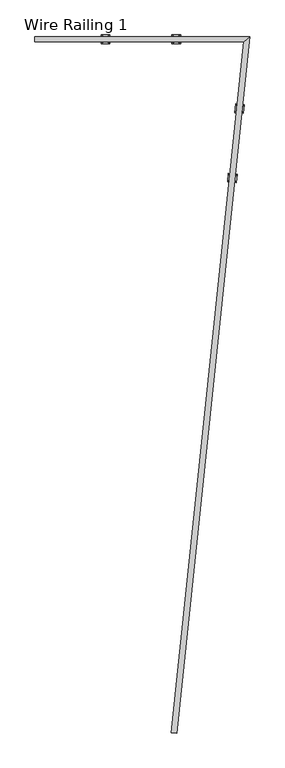
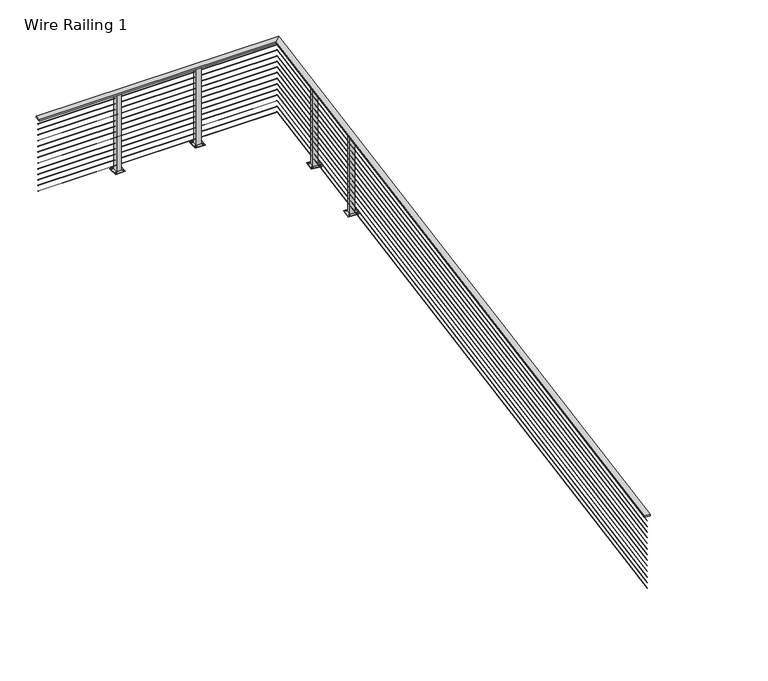
"""IFC4 building model written with IfcOpenShell, lengths in millimetres: railing geometry, Wire Railing 1."""

from ifc_helpers import new_model, si_unit, point, frame, frame_2d, origin, place, context, project, spatial, polyline, circle_curve, ellipse_curve, trimmed, segment, composite_curve, outline, extrude, faceted_brep, source, transform, mapped, element, save
from ifc_brep_helpers import plane_surface, cylinder_surface, advanced_brep


def wire_railing_1_cf5217c8(model_context):
    return source(origin(), model_context, "Body", "SolidModel", [
        faceted_brep([(32254.6127201, 40849.4411612, 270325.85), (32254.6127201, 40925.6411612, 270325.85), (32254.6127201, 40925.6411612, 270306.8), (32254.6127201, 40849.4411612, 270306.8), (35287.8207531, 40849.4411612, 270306.8), (35287.8207531, 40849.4411612, 270325.85), (35372.4494268, 40925.6411612, 270306.8), (35372.4494268, 40925.6411612, 270325.85), (34234.7001024, 30829.6674754, 270325.85), (34234.7001024, 30829.6674754, 270306.8), (34310.4826708, 30821.7024065, 270306.8), (34310.4826708, 30821.7024065, 270325.85)], [[[0, 1, 2, 3]], [[4, 5, 0, 3]], [[6, 4, 3, 2]], [[7, 6, 2, 1]], [[5, 7, 1, 0]], [[8, 9, 10, 11]], [[9, 8, 5, 4]], [[10, 9, 4, 6]], [[11, 10, 6, 7]], [[8, 11, 7, 5]]]),
        advanced_brep(
        [(32254.6127201, 40889.9224112, 270247.26875), (32254.6127201, 40885.1599112, 270247.26875), (35327.4904439, 40885.1599112, 270247.26875), (35332.779736, 40889.9224112, 270247.26875), (34274.9595918, 30825.4360325, 270247.26875), (34270.2231813, 30825.9338493, 270247.26875)],
        [
            (0, 1, circle_curve(frame((32254.6127201, 40887.5411612, 270247.26875), z_axis=(-1.0, 0.0, 0.0), x_axis=(0.0, -1.0, 0.0)), 2.38125)),
            (1, 0, circle_curve(frame((32254.6127201, 40887.5411612, 270247.26875), z_axis=(-1.0, 0.0, 0.0), x_axis=(0.0, -1.0, 0.0)), 2.38125)),
            (2, 3, ellipse_curve(frame((35330.13509, 40887.5411612, 270247.26875), z_axis=(-0.669130606358848, 0.7431448254774035, 0.0), x_axis=(0.7431448254774035, 0.6691306063588481, 0.0)), 3.5587223, 2.38125)),
            (3, 0),
            (1, 2),
            (3, 2, ellipse_curve(frame((35330.13509, 40887.5411612, 270247.26875), z_axis=(-0.669130606358848, 0.7431448254774035, 0.0), x_axis=(0.7431448254774035, 0.6691306063588481, 0.0)), 3.5587223, 2.38125)),
            (4, 5, circle_curve(frame((34272.5913866, 30825.6849409, 270247.26875), z_axis=(-0.10452846326767264, -0.9945218953682714, 0.0), x_axis=(-0.9945218953682714, 0.10452846326767264, 0.0)), 2.38125)),
            (5, 4, circle_curve(frame((34272.5913866, 30825.6849409, 270247.26875), z_axis=(-0.10452846326767264, -0.9945218953682714, 0.0), x_axis=(-0.9945218953682714, 0.10452846326767264, 0.0)), 2.38125)),
            (4, 3),
            (2, 5),
        ],
        [
            plane_surface(frame((32254.6127201, 40887.5411612, 270249.65), z_axis=(-1.0, 0.0, 0.0), x_axis=(0.0, -1.0, 0.0))),
            cylinder_surface(frame((35330.13509, 40887.5411612, 270247.26875), z_axis=(1.0, 0.0, 0.0), x_axis=(0.0, -1.0, 0.0)), 2.38125),
            plane_surface(frame((34272.5913866, 30825.6849409, 270249.65), z_axis=(-0.10452846326767265, -0.9945218953682714, 0.0), x_axis=(0.9945218953682714, -0.10452846326767265, 0.0))),
            cylinder_surface(frame((34272.5913866, 30825.6849409, 270247.26875), z_axis=(-0.10452846326767264, -0.9945218953682714, 0.0), x_axis=(-0.9945218953682714, 0.10452846326767264, 0.0)), 2.38125),
        ],
        [
            (0, [[1, 2]]),
            (1, [[3, 4, -2, 5]]),
            (1, [[6, -5, -1, -4]]),
            (2, [[7, 8]]),
            (3, [[-7, 9, -3, 10]]),
            (3, [[-8, -10, -6, -9]]),
        ],
    ),
        advanced_brep(
        [(32254.6127201, 40889.9224112, 270171.06875), (32254.6127201, 40885.1599112, 270171.06875), (35327.4904439, 40885.1599112, 270171.06875), (35332.779736, 40889.9224112, 270171.06875), (34274.9595918, 30825.4360325, 270171.06875), (34270.2231813, 30825.9338493, 270171.06875)],
        [
            (0, 1, circle_curve(frame((32254.6127201, 40887.5411612, 270171.06875), z_axis=(-1.0, 0.0, 0.0), x_axis=(0.0, -1.0, 0.0)), 2.38125)),
            (1, 0, circle_curve(frame((32254.6127201, 40887.5411612, 270171.06875), z_axis=(-1.0, 0.0, 0.0), x_axis=(0.0, -1.0, 0.0)), 2.38125)),
            (2, 3, ellipse_curve(frame((35330.13509, 40887.5411612, 270171.06875), z_axis=(-0.669130606358848, 0.7431448254774035, 0.0), x_axis=(0.7431448254774035, 0.6691306063588481, 0.0)), 3.5587223, 2.38125)),
            (3, 0),
            (1, 2),
            (3, 2, ellipse_curve(frame((35330.13509, 40887.5411612, 270171.06875), z_axis=(-0.669130606358848, 0.7431448254774035, 0.0), x_axis=(0.7431448254774035, 0.6691306063588481, 0.0)), 3.5587223, 2.38125)),
            (4, 5, circle_curve(frame((34272.5913866, 30825.6849409, 270171.06875), z_axis=(-0.10452846326767264, -0.9945218953682714, 0.0), x_axis=(-0.9945218953682714, 0.10452846326767264, 0.0)), 2.38125)),
            (5, 4, circle_curve(frame((34272.5913866, 30825.6849409, 270171.06875), z_axis=(-0.10452846326767264, -0.9945218953682714, 0.0), x_axis=(-0.9945218953682714, 0.10452846326767264, 0.0)), 2.38125)),
            (4, 3),
            (2, 5),
        ],
        [
            plane_surface(frame((32254.6127201, 40887.5411612, 270173.45), z_axis=(-1.0, 0.0, 0.0), x_axis=(0.0, -1.0, 0.0))),
            cylinder_surface(frame((35330.13509, 40887.5411612, 270171.06875), z_axis=(1.0, 0.0, 0.0), x_axis=(0.0, -1.0, 0.0)), 2.38125),
            plane_surface(frame((34272.5913866, 30825.6849409, 270173.45), z_axis=(-0.10452846326767265, -0.9945218953682714, 0.0), x_axis=(0.9945218953682714, -0.10452846326767265, 0.0))),
            cylinder_surface(frame((34272.5913866, 30825.6849409, 270171.06875), z_axis=(-0.10452846326767264, -0.9945218953682714, 0.0), x_axis=(-0.9945218953682714, 0.10452846326767264, 0.0)), 2.38125),
        ],
        [
            (0, [[1, 2]]),
            (1, [[3, 4, -2, 5]]),
            (1, [[6, -5, -1, -4]]),
            (2, [[7, 8]]),
            (3, [[-7, 9, -3, 10]]),
            (3, [[-8, -10, -6, -9]]),
        ],
    ),
        advanced_brep(
        [(32254.6127201, 40889.9224112, 270094.86875), (32254.6127201, 40885.1599112, 270094.86875), (35327.4904439, 40885.1599112, 270094.86875), (35332.779736, 40889.9224112, 270094.86875), (34274.9595918, 30825.4360325, 270094.86875), (34270.2231813, 30825.9338493, 270094.86875)],
        [
            (0, 1, circle_curve(frame((32254.6127201, 40887.5411612, 270094.86875), z_axis=(-1.0, 0.0, 0.0), x_axis=(0.0, -1.0, 0.0)), 2.38125)),
            (1, 0, circle_curve(frame((32254.6127201, 40887.5411612, 270094.86875), z_axis=(-1.0, 0.0, 0.0), x_axis=(0.0, -1.0, 0.0)), 2.38125)),
            (2, 3, ellipse_curve(frame((35330.13509, 40887.5411612, 270094.86875), z_axis=(-0.669130606358848, 0.7431448254774035, 0.0), x_axis=(0.7431448254774035, 0.6691306063588481, 0.0)), 3.5587223, 2.38125)),
            (3, 0),
            (1, 2),
            (3, 2, ellipse_curve(frame((35330.13509, 40887.5411612, 270094.86875), z_axis=(-0.669130606358848, 0.7431448254774035, 0.0), x_axis=(0.7431448254774035, 0.6691306063588481, 0.0)), 3.5587223, 2.38125)),
            (4, 5, circle_curve(frame((34272.5913866, 30825.6849409, 270094.86875), z_axis=(-0.10452846326767264, -0.9945218953682714, 0.0), x_axis=(-0.9945218953682714, 0.10452846326767264, 0.0)), 2.38125)),
            (5, 4, circle_curve(frame((34272.5913866, 30825.6849409, 270094.86875), z_axis=(-0.10452846326767264, -0.9945218953682714, 0.0), x_axis=(-0.9945218953682714, 0.10452846326767264, 0.0)), 2.38125)),
            (4, 3),
            (2, 5),
        ],
        [
            plane_surface(frame((32254.6127201, 40887.5411612, 270097.25), z_axis=(-1.0, 0.0, 0.0), x_axis=(0.0, -1.0, 0.0))),
            cylinder_surface(frame((35330.13509, 40887.5411612, 270094.86875), z_axis=(1.0, 0.0, 0.0), x_axis=(0.0, -1.0, 0.0)), 2.38125),
            plane_surface(frame((34272.5913866, 30825.6849409, 270097.25), z_axis=(-0.10452846326767265, -0.9945218953682714, 0.0), x_axis=(0.9945218953682714, -0.10452846326767265, 0.0))),
            cylinder_surface(frame((34272.5913866, 30825.6849409, 270094.86875), z_axis=(-0.10452846326767264, -0.9945218953682714, 0.0), x_axis=(-0.9945218953682714, 0.10452846326767264, 0.0)), 2.38125),
        ],
        [
            (0, [[1, 2]]),
            (1, [[3, 4, -2, 5]]),
            (1, [[6, -5, -1, -4]]),
            (2, [[7, 8]]),
            (3, [[-7, 9, -3, 10]]),
            (3, [[-8, -10, -6, -9]]),
        ],
    ),
        advanced_brep(
        [(32254.6127201, 40889.9224112, 270018.66875), (32254.6127201, 40885.1599112, 270018.66875), (35327.4904439, 40885.1599112, 270018.66875), (35332.779736, 40889.9224112, 270018.66875), (34274.9595918, 30825.4360325, 270018.66875), (34270.2231813, 30825.9338493, 270018.66875)],
        [
            (0, 1, circle_curve(frame((32254.6127201, 40887.5411612, 270018.66875), z_axis=(-1.0, 0.0, 0.0), x_axis=(0.0, -1.0, 0.0)), 2.38125)),
            (1, 0, circle_curve(frame((32254.6127201, 40887.5411612, 270018.66875), z_axis=(-1.0, 0.0, 0.0), x_axis=(0.0, -1.0, 0.0)), 2.38125)),
            (2, 3, ellipse_curve(frame((35330.13509, 40887.5411612, 270018.66875), z_axis=(-0.669130606358848, 0.7431448254774035, 0.0), x_axis=(0.7431448254774035, 0.6691306063588481, 0.0)), 3.5587223, 2.38125)),
            (3, 0),
            (1, 2),
            (3, 2, ellipse_curve(frame((35330.13509, 40887.5411612, 270018.66875), z_axis=(-0.669130606358848, 0.7431448254774035, 0.0), x_axis=(0.7431448254774035, 0.6691306063588481, 0.0)), 3.5587223, 2.38125)),
            (4, 5, circle_curve(frame((34272.5913866, 30825.6849409, 270018.66875), z_axis=(-0.10452846326767264, -0.9945218953682714, 0.0), x_axis=(-0.9945218953682714, 0.10452846326767264, 0.0)), 2.38125)),
            (5, 4, circle_curve(frame((34272.5913866, 30825.6849409, 270018.66875), z_axis=(-0.10452846326767264, -0.9945218953682714, 0.0), x_axis=(-0.9945218953682714, 0.10452846326767264, 0.0)), 2.38125)),
            (4, 3),
            (2, 5),
        ],
        [
            plane_surface(frame((32254.6127201, 40887.5411612, 270021.05), z_axis=(-1.0, 0.0, 0.0), x_axis=(0.0, -1.0, 0.0))),
            cylinder_surface(frame((35330.13509, 40887.5411612, 270018.66875), z_axis=(1.0, 0.0, 0.0), x_axis=(0.0, -1.0, 0.0)), 2.38125),
            plane_surface(frame((34272.5913866, 30825.6849409, 270021.05), z_axis=(-0.10452846326767265, -0.9945218953682714, 0.0), x_axis=(0.9945218953682714, -0.10452846326767265, 0.0))),
            cylinder_surface(frame((34272.5913866, 30825.6849409, 270018.66875), z_axis=(-0.10452846326767264, -0.9945218953682714, 0.0), x_axis=(-0.9945218953682714, 0.10452846326767264, 0.0)), 2.38125),
        ],
        [
            (0, [[1, 2]]),
            (1, [[3, 4, -2, 5]]),
            (1, [[6, -5, -1, -4]]),
            (2, [[7, 8]]),
            (3, [[-7, 9, -3, 10]]),
            (3, [[-8, -10, -6, -9]]),
        ],
    ),
        advanced_brep(
        [(32254.6127201, 40889.9224112, 269942.46875), (32254.6127201, 40885.1599112, 269942.46875), (35327.4904439, 40885.1599112, 269942.46875), (35332.779736, 40889.9224112, 269942.46875), (34274.9595918, 30825.4360325, 269942.46875), (34270.2231813, 30825.9338493, 269942.46875)],
        [
            (0, 1, circle_curve(frame((32254.6127201, 40887.5411612, 269942.46875), z_axis=(-1.0, 0.0, 0.0), x_axis=(0.0, -1.0, 0.0)), 2.38125)),
            (1, 0, circle_curve(frame((32254.6127201, 40887.5411612, 269942.46875), z_axis=(-1.0, 0.0, 0.0), x_axis=(0.0, -1.0, 0.0)), 2.38125)),
            (2, 3, ellipse_curve(frame((35330.13509, 40887.5411612, 269942.46875), z_axis=(-0.669130606358848, 0.7431448254774035, 0.0), x_axis=(0.7431448254774035, 0.6691306063588481, 0.0)), 3.5587223, 2.38125)),
            (3, 0),
            (1, 2),
            (3, 2, ellipse_curve(frame((35330.13509, 40887.5411612, 269942.46875), z_axis=(-0.669130606358848, 0.7431448254774035, 0.0), x_axis=(0.7431448254774035, 0.6691306063588481, 0.0)), 3.5587223, 2.38125)),
            (4, 5, circle_curve(frame((34272.5913866, 30825.6849409, 269942.46875), z_axis=(-0.10452846326767264, -0.9945218953682714, 0.0), x_axis=(-0.9945218953682714, 0.10452846326767264, 0.0)), 2.38125)),
            (5, 4, circle_curve(frame((34272.5913866, 30825.6849409, 269942.46875), z_axis=(-0.10452846326767264, -0.9945218953682714, 0.0), x_axis=(-0.9945218953682714, 0.10452846326767264, 0.0)), 2.38125)),
            (4, 3),
            (2, 5),
        ],
        [
            plane_surface(frame((32254.6127201, 40887.5411612, 269944.85), z_axis=(-1.0, 0.0, 0.0), x_axis=(0.0, -1.0, 0.0))),
            cylinder_surface(frame((35330.13509, 40887.5411612, 269942.46875), z_axis=(1.0, 0.0, 0.0), x_axis=(0.0, -1.0, 0.0)), 2.38125),
            plane_surface(frame((34272.5913866, 30825.6849409, 269944.85), z_axis=(-0.10452846326767265, -0.9945218953682714, 0.0), x_axis=(0.9945218953682714, -0.10452846326767265, 0.0))),
            cylinder_surface(frame((34272.5913866, 30825.6849409, 269942.46875), z_axis=(-0.10452846326767264, -0.9945218953682714, 0.0), x_axis=(-0.9945218953682714, 0.10452846326767264, 0.0)), 2.38125),
        ],
        [
            (0, [[1, 2]]),
            (1, [[3, 4, -2, 5]]),
            (1, [[6, -5, -1, -4]]),
            (2, [[7, 8]]),
            (3, [[-7, 9, -3, 10]]),
            (3, [[-8, -10, -6, -9]]),
        ],
    ),
        advanced_brep(
        [(32254.6127201, 40889.9224112, 269866.26875), (32254.6127201, 40885.1599112, 269866.26875), (35327.4904439, 40885.1599112, 269866.26875), (35332.779736, 40889.9224112, 269866.26875), (34274.9595918, 30825.4360325, 269866.26875), (34270.2231813, 30825.9338493, 269866.26875)],
        [
            (0, 1, circle_curve(frame((32254.6127201, 40887.5411612, 269866.26875), z_axis=(-1.0, 0.0, 0.0), x_axis=(0.0, -1.0, 0.0)), 2.38125)),
            (1, 0, circle_curve(frame((32254.6127201, 40887.5411612, 269866.26875), z_axis=(-1.0, 0.0, 0.0), x_axis=(0.0, -1.0, 0.0)), 2.38125)),
            (2, 3, ellipse_curve(frame((35330.13509, 40887.5411612, 269866.26875), z_axis=(-0.669130606358848, 0.7431448254774035, 0.0), x_axis=(0.7431448254774035, 0.6691306063588481, 0.0)), 3.5587223, 2.38125)),
            (3, 0),
            (1, 2),
            (3, 2, ellipse_curve(frame((35330.13509, 40887.5411612, 269866.26875), z_axis=(-0.669130606358848, 0.7431448254774035, 0.0), x_axis=(0.7431448254774035, 0.6691306063588481, 0.0)), 3.5587223, 2.38125)),
            (4, 5, circle_curve(frame((34272.5913866, 30825.6849409, 269866.26875), z_axis=(-0.10452846326767264, -0.9945218953682714, 0.0), x_axis=(-0.9945218953682714, 0.10452846326767264, 0.0)), 2.38125)),
            (5, 4, circle_curve(frame((34272.5913866, 30825.6849409, 269866.26875), z_axis=(-0.10452846326767264, -0.9945218953682714, 0.0), x_axis=(-0.9945218953682714, 0.10452846326767264, 0.0)), 2.38125)),
            (4, 3),
            (2, 5),
        ],
        [
            plane_surface(frame((32254.6127201, 40887.5411612, 269868.65), z_axis=(-1.0, 0.0, 0.0), x_axis=(0.0, -1.0, 0.0))),
            cylinder_surface(frame((35330.13509, 40887.5411612, 269866.26875), z_axis=(1.0, 0.0, 0.0), x_axis=(0.0, -1.0, 0.0)), 2.38125),
            plane_surface(frame((34272.5913866, 30825.6849409, 269868.65), z_axis=(-0.10452846326767265, -0.9945218953682714, 0.0), x_axis=(0.9945218953682714, -0.10452846326767265, 0.0))),
            cylinder_surface(frame((34272.5913866, 30825.6849409, 269866.26875), z_axis=(-0.10452846326767264, -0.9945218953682714, 0.0), x_axis=(-0.9945218953682714, 0.10452846326767264, 0.0)), 2.38125),
        ],
        [
            (0, [[1, 2]]),
            (1, [[3, 4, -2, 5]]),
            (1, [[6, -5, -1, -4]]),
            (2, [[7, 8]]),
            (3, [[-7, 9, -3, 10]]),
            (3, [[-8, -10, -6, -9]]),
        ],
    ),
        advanced_brep(
        [(32254.6127201, 40889.9224112, 269790.06875), (32254.6127201, 40885.1599112, 269790.06875), (35327.4904439, 40885.1599112, 269790.06875), (35332.779736, 40889.9224112, 269790.06875), (34274.9595918, 30825.4360325, 269790.06875), (34270.2231813, 30825.9338493, 269790.06875)],
        [
            (0, 1, circle_curve(frame((32254.6127201, 40887.5411612, 269790.06875), z_axis=(-1.0, 0.0, 0.0), x_axis=(0.0, -1.0, 0.0)), 2.38125)),
            (1, 0, circle_curve(frame((32254.6127201, 40887.5411612, 269790.06875), z_axis=(-1.0, 0.0, 0.0), x_axis=(0.0, -1.0, 0.0)), 2.38125)),
            (2, 3, ellipse_curve(frame((35330.13509, 40887.5411612, 269790.06875), z_axis=(-0.669130606358848, 0.7431448254774035, 0.0), x_axis=(0.7431448254774035, 0.6691306063588481, 0.0)), 3.5587223, 2.38125)),
            (3, 0),
            (1, 2),
            (3, 2, ellipse_curve(frame((35330.13509, 40887.5411612, 269790.06875), z_axis=(-0.669130606358848, 0.7431448254774035, 0.0), x_axis=(0.7431448254774035, 0.6691306063588481, 0.0)), 3.5587223, 2.38125)),
            (4, 5, circle_curve(frame((34272.5913866, 30825.6849409, 269790.06875), z_axis=(-0.10452846326767264, -0.9945218953682714, 0.0), x_axis=(-0.9945218953682714, 0.10452846326767264, 0.0)), 2.38125)),
            (5, 4, circle_curve(frame((34272.5913866, 30825.6849409, 269790.06875), z_axis=(-0.10452846326767264, -0.9945218953682714, 0.0), x_axis=(-0.9945218953682714, 0.10452846326767264, 0.0)), 2.38125)),
            (4, 3),
            (2, 5),
        ],
        [
            plane_surface(frame((32254.6127201, 40887.5411612, 269792.45), z_axis=(-1.0, 0.0, 0.0), x_axis=(0.0, -1.0, 0.0))),
            cylinder_surface(frame((35330.13509, 40887.5411612, 269790.06875), z_axis=(1.0, 0.0, 0.0), x_axis=(0.0, -1.0, 0.0)), 2.38125),
            plane_surface(frame((34272.5913866, 30825.6849409, 269792.45), z_axis=(-0.10452846326767265, -0.9945218953682714, 0.0), x_axis=(0.9945218953682714, -0.10452846326767265, 0.0))),
            cylinder_surface(frame((34272.5913866, 30825.6849409, 269790.06875), z_axis=(-0.10452846326767264, -0.9945218953682714, 0.0), x_axis=(-0.9945218953682714, 0.10452846326767264, 0.0)), 2.38125),
        ],
        [
            (0, [[1, 2]]),
            (1, [[3, 4, -2, 5]]),
            (1, [[6, -5, -1, -4]]),
            (2, [[7, 8]]),
            (3, [[-7, 9, -3, 10]]),
            (3, [[-8, -10, -6, -9]]),
        ],
    ),
        advanced_brep(
        [(32254.6127201, 40889.9224112, 269713.86875), (32254.6127201, 40885.1599112, 269713.86875), (35327.4904439, 40885.1599112, 269713.86875), (35332.779736, 40889.9224112, 269713.86875), (34274.9595918, 30825.4360325, 269713.86875), (34270.2231813, 30825.9338493, 269713.86875)],
        [
            (0, 1, circle_curve(frame((32254.6127201, 40887.5411612, 269713.86875), z_axis=(-1.0, 0.0, 0.0), x_axis=(0.0, -1.0, 0.0)), 2.38125)),
            (1, 0, circle_curve(frame((32254.6127201, 40887.5411612, 269713.86875), z_axis=(-1.0, 0.0, 0.0), x_axis=(0.0, -1.0, 0.0)), 2.38125)),
            (2, 3, ellipse_curve(frame((35330.13509, 40887.5411612, 269713.86875), z_axis=(-0.669130606358848, 0.7431448254774035, 0.0), x_axis=(0.7431448254774035, 0.6691306063588481, 0.0)), 3.5587223, 2.38125)),
            (3, 0),
            (1, 2),
            (3, 2, ellipse_curve(frame((35330.13509, 40887.5411612, 269713.86875), z_axis=(-0.669130606358848, 0.7431448254774035, 0.0), x_axis=(0.7431448254774035, 0.6691306063588481, 0.0)), 3.5587223, 2.38125)),
            (4, 5, circle_curve(frame((34272.5913866, 30825.6849409, 269713.86875), z_axis=(-0.10452846326767264, -0.9945218953682714, 0.0), x_axis=(-0.9945218953682714, 0.10452846326767264, 0.0)), 2.38125)),
            (5, 4, circle_curve(frame((34272.5913866, 30825.6849409, 269713.86875), z_axis=(-0.10452846326767264, -0.9945218953682714, 0.0), x_axis=(-0.9945218953682714, 0.10452846326767264, 0.0)), 2.38125)),
            (4, 3),
            (2, 5),
        ],
        [
            plane_surface(frame((32254.6127201, 40887.5411612, 269716.25), z_axis=(-1.0, 0.0, 0.0), x_axis=(0.0, -1.0, 0.0))),
            cylinder_surface(frame((35330.13509, 40887.5411612, 269713.86875), z_axis=(1.0, 0.0, 0.0), x_axis=(0.0, -1.0, 0.0)), 2.38125),
            plane_surface(frame((34272.5913866, 30825.6849409, 269716.25), z_axis=(-0.10452846326767265, -0.9945218953682714, 0.0), x_axis=(0.9945218953682714, -0.10452846326767265, 0.0))),
            cylinder_surface(frame((34272.5913866, 30825.6849409, 269713.86875), z_axis=(-0.10452846326767264, -0.9945218953682714, 0.0), x_axis=(-0.9945218953682714, 0.10452846326767264, 0.0)), 2.38125),
        ],
        [
            (0, [[1, 2]]),
            (1, [[3, 4, -2, 5]]),
            (1, [[6, -5, -1, -4]]),
            (2, [[7, 8]]),
            (3, [[-7, 9, -3, 10]]),
            (3, [[-8, -10, -6, -9]]),
        ],
    ),
        advanced_brep(
        [(32254.6127201, 40889.9224112, 269637.66875), (32254.6127201, 40885.1599112, 269637.66875), (35327.4904439, 40885.1599112, 269637.66875), (35332.779736, 40889.9224112, 269637.66875), (34274.9595918, 30825.4360325, 269637.66875), (34270.2231813, 30825.9338493, 269637.66875)],
        [
            (0, 1, circle_curve(frame((32254.6127201, 40887.5411612, 269637.66875), z_axis=(-1.0, 0.0, 0.0), x_axis=(0.0, -1.0, 0.0)), 2.38125)),
            (1, 0, circle_curve(frame((32254.6127201, 40887.5411612, 269637.66875), z_axis=(-1.0, 0.0, 0.0), x_axis=(0.0, -1.0, 0.0)), 2.38125)),
            (2, 3, ellipse_curve(frame((35330.13509, 40887.5411612, 269637.66875), z_axis=(-0.669130606358848, 0.7431448254774035, 0.0), x_axis=(0.7431448254774035, 0.6691306063588481, 0.0)), 3.5587223, 2.38125)),
            (3, 0),
            (1, 2),
            (3, 2, ellipse_curve(frame((35330.13509, 40887.5411612, 269637.66875), z_axis=(-0.669130606358848, 0.7431448254774035, 0.0), x_axis=(0.7431448254774035, 0.6691306063588481, 0.0)), 3.5587223, 2.38125)),
            (4, 5, circle_curve(frame((34272.5913866, 30825.6849409, 269637.66875), z_axis=(-0.10452846326767264, -0.9945218953682714, 0.0), x_axis=(-0.9945218953682714, 0.10452846326767264, 0.0)), 2.38125)),
            (5, 4, circle_curve(frame((34272.5913866, 30825.6849409, 269637.66875), z_axis=(-0.10452846326767264, -0.9945218953682714, 0.0), x_axis=(-0.9945218953682714, 0.10452846326767264, 0.0)), 2.38125)),
            (4, 3),
            (2, 5),
        ],
        [
            plane_surface(frame((32254.6127201, 40887.5411612, 269640.05), z_axis=(-1.0, 0.0, 0.0), x_axis=(0.0, -1.0, 0.0))),
            cylinder_surface(frame((35330.13509, 40887.5411612, 269637.66875), z_axis=(1.0, 0.0, 0.0), x_axis=(0.0, -1.0, 0.0)), 2.38125),
            plane_surface(frame((34272.5913866, 30825.6849409, 269640.05), z_axis=(-0.10452846326767265, -0.9945218953682714, 0.0), x_axis=(0.9945218953682714, -0.10452846326767265, 0.0))),
            cylinder_surface(frame((34272.5913866, 30825.6849409, 269637.66875), z_axis=(-0.10452846326767264, -0.9945218953682714, 0.0), x_axis=(-0.9945218953682714, 0.10452846326767264, 0.0)), 2.38125),
        ],
        [
            (0, [[1, 2]]),
            (1, [[3, 4, -2, 5]]),
            (1, [[6, -5, -1, -4]]),
            (2, [[7, 8]]),
            (3, [[-7, 9, -3, 10]]),
            (3, [[-8, -10, -6, -9]]),
        ],
    ),
        advanced_brep(
        [(32254.6127201, 40889.9224112, 269561.46875), (32254.6127201, 40885.1599112, 269561.46875), (35327.4904439, 40885.1599112, 269561.46875), (35332.779736, 40889.9224112, 269561.46875), (34274.9595918, 30825.4360325, 269561.46875), (34270.2231813, 30825.9338493, 269561.46875)],
        [
            (0, 1, circle_curve(frame((32254.6127201, 40887.5411612, 269561.46875), z_axis=(-1.0, 0.0, 0.0), x_axis=(0.0, -1.0, 0.0)), 2.38125)),
            (1, 0, circle_curve(frame((32254.6127201, 40887.5411612, 269561.46875), z_axis=(-1.0, 0.0, 0.0), x_axis=(0.0, -1.0, 0.0)), 2.38125)),
            (2, 3, ellipse_curve(frame((35330.13509, 40887.5411612, 269561.46875), z_axis=(-0.669130606358848, 0.7431448254774035, 0.0), x_axis=(0.7431448254774035, 0.6691306063588481, 0.0)), 3.5587223, 2.38125)),
            (3, 0),
            (1, 2),
            (3, 2, ellipse_curve(frame((35330.13509, 40887.5411612, 269561.46875), z_axis=(-0.669130606358848, 0.7431448254774035, 0.0), x_axis=(0.7431448254774035, 0.6691306063588481, 0.0)), 3.5587223, 2.38125)),
            (4, 5, circle_curve(frame((34272.5913866, 30825.6849409, 269561.46875), z_axis=(-0.10452846326767264, -0.9945218953682714, 0.0), x_axis=(-0.9945218953682714, 0.10452846326767264, 0.0)), 2.38125)),
            (5, 4, circle_curve(frame((34272.5913866, 30825.6849409, 269561.46875), z_axis=(-0.10452846326767264, -0.9945218953682714, 0.0), x_axis=(-0.9945218953682714, 0.10452846326767264, 0.0)), 2.38125)),
            (4, 3),
            (2, 5),
        ],
        [
            plane_surface(frame((32254.6127201, 40887.5411612, 269563.85), z_axis=(-1.0, 0.0, 0.0), x_axis=(0.0, -1.0, 0.0))),
            cylinder_surface(frame((35330.13509, 40887.5411612, 269561.46875), z_axis=(1.0, 0.0, 0.0), x_axis=(0.0, -1.0, 0.0)), 2.38125),
            plane_surface(frame((34272.5913866, 30825.6849409, 269563.85), z_axis=(-0.10452846326767265, -0.9945218953682714, 0.0), x_axis=(0.9945218953682714, -0.10452846326767265, 0.0))),
            cylinder_surface(frame((34272.5913866, 30825.6849409, 269561.46875), z_axis=(-0.10452846326767264, -0.9945218953682714, 0.0), x_axis=(-0.9945218953682714, 0.10452846326767264, 0.0)), 2.38125),
        ],
        [
            (0, [[1, 2]]),
            (1, [[3, 4, -2, 5]]),
            (1, [[6, -5, -1, -4]]),
            (2, [[7, 8]]),
            (3, [[-7, 9, -3, 10]]),
            (3, [[-8, -10, -6, -9]]),
        ],
    ),
        advanced_brep(
        [(32254.6127201, 40889.9224112, 269485.26875), (32254.6127201, 40885.1599112, 269485.26875), (35327.4904439, 40885.1599112, 269485.26875), (35332.779736, 40889.9224112, 269485.26875), (34274.9595918, 30825.4360325, 269485.26875), (34270.2231813, 30825.9338493, 269485.26875)],
        [
            (0, 1, circle_curve(frame((32254.6127201, 40887.5411612, 269485.26875), z_axis=(-1.0, 0.0, 0.0), x_axis=(0.0, -1.0, 0.0)), 2.38125)),
            (1, 0, circle_curve(frame((32254.6127201, 40887.5411612, 269485.26875), z_axis=(-1.0, 0.0, 0.0), x_axis=(0.0, -1.0, 0.0)), 2.38125)),
            (2, 3, ellipse_curve(frame((35330.13509, 40887.5411612, 269485.26875), z_axis=(-0.669130606358848, 0.7431448254774035, 0.0), x_axis=(0.7431448254774035, 0.6691306063588481, 0.0)), 3.5587223, 2.38125)),
            (3, 0),
            (1, 2),
            (3, 2, ellipse_curve(frame((35330.13509, 40887.5411612, 269485.26875), z_axis=(-0.669130606358848, 0.7431448254774035, 0.0), x_axis=(0.7431448254774035, 0.6691306063588481, 0.0)), 3.5587223, 2.38125)),
            (4, 5, circle_curve(frame((34272.5913866, 30825.6849409, 269485.26875), z_axis=(-0.10452846326767264, -0.9945218953682714, 0.0), x_axis=(-0.9945218953682714, 0.10452846326767264, 0.0)), 2.38125)),
            (5, 4, circle_curve(frame((34272.5913866, 30825.6849409, 269485.26875), z_axis=(-0.10452846326767264, -0.9945218953682714, 0.0), x_axis=(-0.9945218953682714, 0.10452846326767264, 0.0)), 2.38125)),
            (4, 3),
            (2, 5),
        ],
        [
            plane_surface(frame((32254.6127201, 40887.5411612, 269487.65), z_axis=(-1.0, 0.0, 0.0), x_axis=(0.0, -1.0, 0.0))),
            cylinder_surface(frame((35330.13509, 40887.5411612, 269485.26875), z_axis=(1.0, 0.0, 0.0), x_axis=(0.0, -1.0, 0.0)), 2.38125),
            plane_surface(frame((34272.5913866, 30825.6849409, 269487.65), z_axis=(-0.10452846326767265, -0.9945218953682714, 0.0), x_axis=(0.9945218953682714, -0.10452846326767265, 0.0))),
            cylinder_surface(frame((34272.5913866, 30825.6849409, 269485.26875), z_axis=(-0.10452846326767264, -0.9945218953682714, 0.0), x_axis=(-0.9945218953682714, 0.10452846326767264, 0.0)), 2.38125),
        ],
        [
            (0, [[1, 2]]),
            (1, [[3, 4, -2, 5]]),
            (1, [[6, -5, -1, -4]]),
            (2, [[7, 8]]),
            (3, [[-7, 9, -3, 10]]),
            (3, [[-8, -10, -6, -9]]),
        ],
    ),
        advanced_brep(
        [(32254.6127201, 40889.9224112, 269409.06875), (32254.6127201, 40885.1599112, 269409.06875), (35327.4904439, 40885.1599112, 269409.06875), (35332.779736, 40889.9224112, 269409.06875), (34274.9595918, 30825.4360325, 269409.06875), (34270.2231813, 30825.9338493, 269409.06875)],
        [
            (0, 1, circle_curve(frame((32254.6127201, 40887.5411612, 269409.06875), z_axis=(-1.0, 0.0, 0.0), x_axis=(0.0, -1.0, 0.0)), 2.38125)),
            (1, 0, circle_curve(frame((32254.6127201, 40887.5411612, 269409.06875), z_axis=(-1.0, 0.0, 0.0), x_axis=(0.0, -1.0, 0.0)), 2.38125)),
            (2, 3, ellipse_curve(frame((35330.13509, 40887.5411612, 269409.06875), z_axis=(-0.669130606358848, 0.7431448254774035, 0.0), x_axis=(0.7431448254774035, 0.6691306063588481, 0.0)), 3.5587223, 2.38125)),
            (3, 0),
            (1, 2),
            (3, 2, ellipse_curve(frame((35330.13509, 40887.5411612, 269409.06875), z_axis=(-0.669130606358848, 0.7431448254774035, 0.0), x_axis=(0.7431448254774035, 0.6691306063588481, 0.0)), 3.5587223, 2.38125)),
            (4, 5, circle_curve(frame((34272.5913866, 30825.6849409, 269409.06875), z_axis=(-0.10452846326767264, -0.9945218953682714, 0.0), x_axis=(-0.9945218953682714, 0.10452846326767264, 0.0)), 2.38125)),
            (5, 4, circle_curve(frame((34272.5913866, 30825.6849409, 269409.06875), z_axis=(-0.10452846326767264, -0.9945218953682714, 0.0), x_axis=(-0.9945218953682714, 0.10452846326767264, 0.0)), 2.38125)),
            (4, 3),
            (2, 5),
        ],
        [
            plane_surface(frame((32254.6127201, 40887.5411612, 269411.45), z_axis=(-1.0, 0.0, 0.0), x_axis=(0.0, -1.0, 0.0))),
            cylinder_surface(frame((35330.13509, 40887.5411612, 269409.06875), z_axis=(1.0, 0.0, 0.0), x_axis=(0.0, -1.0, 0.0)), 2.38125),
            plane_surface(frame((34272.5913866, 30825.6849409, 269411.45), z_axis=(-0.10452846326767265, -0.9945218953682714, 0.0), x_axis=(0.9945218953682714, -0.10452846326767265, 0.0))),
            cylinder_surface(frame((34272.5913866, 30825.6849409, 269409.06875), z_axis=(-0.10452846326767264, -0.9945218953682714, 0.0), x_axis=(-0.9945218953682714, 0.10452846326767264, 0.0)), 2.38125),
        ],
        [
            (0, [[1, 2]]),
            (1, [[3, 4, -2, 5]]),
            (1, [[6, -5, -1, -4]]),
            (2, [[7, 8]]),
            (3, [[-7, 9, -3, 10]]),
            (3, [[-8, -10, -6, -9]]),
        ],
    ),
        advanced_brep(
        [(32254.6127201, 40889.9224112, 269332.86875), (32254.6127201, 40885.1599112, 269332.86875), (35327.4904439, 40885.1599112, 269332.86875), (35332.779736, 40889.9224112, 269332.86875), (34274.9595918, 30825.4360325, 269332.86875), (34270.2231813, 30825.9338493, 269332.86875)],
        [
            (0, 1, circle_curve(frame((32254.6127201, 40887.5411612, 269332.86875), z_axis=(-1.0, 0.0, 0.0), x_axis=(0.0, -1.0, 0.0)), 2.38125)),
            (1, 0, circle_curve(frame((32254.6127201, 40887.5411612, 269332.86875), z_axis=(-1.0, 0.0, 0.0), x_axis=(0.0, -1.0, 0.0)), 2.38125)),
            (2, 3, ellipse_curve(frame((35330.13509, 40887.5411612, 269332.86875), z_axis=(-0.669130606358848, 0.7431448254774035, 0.0), x_axis=(0.7431448254774035, 0.6691306063588481, 0.0)), 3.5587223, 2.38125)),
            (3, 0),
            (1, 2),
            (3, 2, ellipse_curve(frame((35330.13509, 40887.5411612, 269332.86875), z_axis=(-0.669130606358848, 0.7431448254774035, 0.0), x_axis=(0.7431448254774035, 0.6691306063588481, 0.0)), 3.5587223, 2.38125)),
            (4, 5, circle_curve(frame((34272.5913866, 30825.6849409, 269332.86875), z_axis=(-0.10452846326767264, -0.9945218953682714, 0.0), x_axis=(-0.9945218953682714, 0.10452846326767264, 0.0)), 2.38125)),
            (5, 4, circle_curve(frame((34272.5913866, 30825.6849409, 269332.86875), z_axis=(-0.10452846326767264, -0.9945218953682714, 0.0), x_axis=(-0.9945218953682714, 0.10452846326767264, 0.0)), 2.38125)),
            (4, 3),
            (2, 5),
        ],
        [
            plane_surface(frame((32254.6127201, 40887.5411612, 269335.25), z_axis=(-1.0, 0.0, 0.0), x_axis=(0.0, -1.0, 0.0))),
            cylinder_surface(frame((35330.13509, 40887.5411612, 269332.86875), z_axis=(1.0, 0.0, 0.0), x_axis=(0.0, -1.0, 0.0)), 2.38125),
            plane_surface(frame((34272.5913866, 30825.6849409, 269335.25), z_axis=(-0.10452846326767265, -0.9945218953682714, 0.0), x_axis=(0.9945218953682714, -0.10452846326767265, 0.0))),
            cylinder_surface(frame((34272.5913866, 30825.6849409, 269332.86875), z_axis=(-0.10452846326767264, -0.9945218953682714, 0.0), x_axis=(-0.9945218953682714, 0.10452846326767264, 0.0)), 2.38125),
        ],
        [
            (0, [[1, 2]]),
            (1, [[3, 4, -2, 5]]),
            (1, [[6, -5, -1, -4]]),
            (2, [[7, 8]]),
            (3, [[-7, 9, -3, 10]]),
            (3, [[-8, -10, -6, -9]]),
        ],
    ),
        extrude(outline(composite_curve([segment(trimmed(circle_curve(frame_2d((33324.2368434, 40843.0911612)), 6.35), [point((33324.2368434, 40836.7411612))], [point((33324.2368434, 40849.4411612))], False, "CARTESIAN"), True, "CONTINUOUS"), segment(trimmed(circle_curve(frame_2d((33324.2368434, 40843.0911612)), 6.35), [point((33324.2368434, 40849.4411612))], [point((33324.2368434, 40836.7411612))], False, "CARTESIAN"), True, "CONTINUOUS")], self_intersect=False)), frame((0.0, 0.0, 269259.05), z_axis=(0.0, 0.0, 1.0), x_axis=(1.0, 0.0, 0.0)), (0.0, 0.0, 1.0), 12.7),
        extrude(outline(composite_curve([segment(trimmed(circle_curve(frame_2d((33324.2368434, 40931.9911612)), 6.35), [point((33324.2368434, 40925.6411612))], [point((33324.2368434, 40938.3411612))], False, "CARTESIAN"), True, "CONTINUOUS"), segment(trimmed(circle_curve(frame_2d((33324.2368434, 40931.9911612)), 6.35), [point((33324.2368434, 40938.3411612))], [point((33324.2368434, 40925.6411612))], False, "CARTESIAN"), True, "CONTINUOUS")], self_intersect=False)), frame((0.0, 0.0, 269259.05), z_axis=(0.0, 0.0, 1.0), x_axis=(1.0, 0.0, 0.0)), (0.0, 0.0, 1.0), 12.7),
        extrude(outline(composite_curve([segment(trimmed(circle_curve(frame_2d((33235.3368434, 40843.0911612)), 6.35), [point((33235.3368434, 40836.7411612))], [point((33235.3368434, 40849.4411612))], False, "CARTESIAN"), True, "CONTINUOUS"), segment(trimmed(circle_curve(frame_2d((33235.3368434, 40843.0911612)), 6.35), [point((33235.3368434, 40849.4411612))], [point((33235.3368434, 40836.7411612))], False, "CARTESIAN"), True, "CONTINUOUS")], self_intersect=False)), frame((0.0, 0.0, 269259.05), z_axis=(0.0, 0.0, 1.0), x_axis=(1.0, 0.0, 0.0)), (0.0, 0.0, 1.0), 12.7),
        extrude(outline(composite_curve([segment(trimmed(circle_curve(frame_2d((33235.3368434, 40931.9911612)), 6.35), [point((33235.3368434, 40925.6411612))], [point((33235.3368434, 40938.3411612))], False, "CARTESIAN"), True, "CONTINUOUS"), segment(trimmed(circle_curve(frame_2d((33235.3368434, 40931.9911612)), 6.35), [point((33235.3368434, 40938.3411612))], [point((33235.3368434, 40925.6411612))], False, "CARTESIAN"), True, "CONTINUOUS")], self_intersect=False)), frame((0.0, 0.0, 269259.05), z_axis=(0.0, 0.0, 1.0), x_axis=(1.0, 0.0, 0.0)), (0.0, 0.0, 1.0), 12.7),
        extrude(outline(polyline([(33343.2868434, 40951.0411612), (33343.2868434, 40824.0411612), (33216.2868434, 40824.0411612), (33216.2868434, 40951.0411612), (33343.2868434, 40951.0411612)])), frame((0.0, 0.0, 269259.05), z_axis=(0.0, 0.0, 1.0), x_axis=(1.0, 0.0, 0.0)), (0.0, 0.0, 1.0), 6.35),
        extrude(outline(polyline([(33309.9493434, 40917.7036612), (33309.9493434, 40857.3786612), (33249.6243434, 40857.3786612), (33249.6243434, 40917.7036612), (33309.9493434, 40917.7036612)]), holes=[polyline([(33303.5993434, 40911.3536612), (33255.9743434, 40911.3536612), (33255.9743434, 40863.7286612), (33303.5993434, 40863.7286612), (33303.5993434, 40911.3536612)])]), frame((0.0, 0.0, 269259.05), z_axis=(0.0, 0.0, 1.0), x_axis=(1.0, 0.0, 0.0)), (0.0, 0.0, 1.0), 1047.75),
        extrude(outline(composite_curve([segment(trimmed(circle_curve(frame_2d((34349.4109667, 40843.0911612)), 6.35), [point((34349.4109667, 40836.7411612))], [point((34349.4109667, 40849.4411612))], False, "CARTESIAN"), True, "CONTINUOUS"), segment(trimmed(circle_curve(frame_2d((34349.4109667, 40843.0911612)), 6.35), [point((34349.4109667, 40849.4411612))], [point((34349.4109667, 40836.7411612))], False, "CARTESIAN"), True, "CONTINUOUS")], self_intersect=False)), frame((0.0, 0.0, 269259.05), z_axis=(0.0, 0.0, 1.0), x_axis=(1.0, 0.0, 0.0)), (0.0, 0.0, 1.0), 12.7),
        extrude(outline(composite_curve([segment(trimmed(circle_curve(frame_2d((34349.4109667, 40931.9911612)), 6.35), [point((34349.4109667, 40925.6411612))], [point((34349.4109667, 40938.3411612))], False, "CARTESIAN"), True, "CONTINUOUS"), segment(trimmed(circle_curve(frame_2d((34349.4109667, 40931.9911612)), 6.35), [point((34349.4109667, 40938.3411612))], [point((34349.4109667, 40925.6411612))], False, "CARTESIAN"), True, "CONTINUOUS")], self_intersect=False)), frame((0.0, 0.0, 269259.05), z_axis=(0.0, 0.0, 1.0), x_axis=(1.0, 0.0, 0.0)), (0.0, 0.0, 1.0), 12.7),
        extrude(outline(composite_curve([segment(trimmed(circle_curve(frame_2d((34260.5109667, 40843.0911612)), 6.35), [point((34260.5109667, 40836.7411612))], [point((34260.5109667, 40849.4411612))], False, "CARTESIAN"), True, "CONTINUOUS"), segment(trimmed(circle_curve(frame_2d((34260.5109667, 40843.0911612)), 6.35), [point((34260.5109667, 40849.4411612))], [point((34260.5109667, 40836.7411612))], False, "CARTESIAN"), True, "CONTINUOUS")], self_intersect=False)), frame((0.0, 0.0, 269259.05), z_axis=(0.0, 0.0, 1.0), x_axis=(1.0, 0.0, 0.0)), (0.0, 0.0, 1.0), 12.7),
        extrude(outline(composite_curve([segment(trimmed(circle_curve(frame_2d((34260.5109667, 40931.9911612)), 6.35), [point((34260.5109667, 40925.6411612))], [point((34260.5109667, 40938.3411612))], False, "CARTESIAN"), True, "CONTINUOUS"), segment(trimmed(circle_curve(frame_2d((34260.5109667, 40931.9911612)), 6.35), [point((34260.5109667, 40938.3411612))], [point((34260.5109667, 40925.6411612))], False, "CARTESIAN"), True, "CONTINUOUS")], self_intersect=False)), frame((0.0, 0.0, 269259.05), z_axis=(0.0, 0.0, 1.0), x_axis=(1.0, 0.0, 0.0)), (0.0, 0.0, 1.0), 12.7),
        extrude(outline(polyline([(34368.4609667, 40951.0411612), (34368.4609667, 40824.0411612), (34241.4609667, 40824.0411612), (34241.4609667, 40951.0411612), (34368.4609667, 40951.0411612)])), frame((0.0, 0.0, 269259.05), z_axis=(0.0, 0.0, 1.0), x_axis=(1.0, 0.0, 0.0)), (0.0, 0.0, 1.0), 6.35),
        extrude(outline(polyline([(34335.1234667, 40917.7036612), (34335.1234667, 40857.3786612), (34274.7984667, 40857.3786612), (34274.7984667, 40917.7036612), (34335.1234667, 40917.7036612)]), holes=[polyline([(34328.7734667, 40911.3536612), (34281.1484667, 40911.3536612), (34281.1484667, 40863.7286612), (34328.7734667, 40863.7286612), (34328.7734667, 40911.3536612)])]), frame((0.0, 0.0, 269259.05), z_axis=(0.0, 0.0, 1.0), x_axis=(1.0, 0.0, 0.0)), (0.0, 0.0, 1.0), 1047.75),
        extrude(outline(composite_curve([segment(trimmed(circle_curve(frame_2d((35175.5279312, 39841.7953311)), 6.35), [point((35169.2127171, 39842.4590869))], [point((35181.8431452, 39841.1315754))], False, "CARTESIAN"), True, "CONTINUOUS"), segment(trimmed(circle_curve(frame_2d((35175.5279312, 39841.7953311)), 6.35), [point((35181.8431452, 39841.1315754))], [point((35169.2127171, 39842.4590869))], False, "CARTESIAN"), True, "CONTINUOUS")], self_intersect=False)), frame((0.0, 0.0, 269259.05), z_axis=(0.0, 0.0, 1.0), x_axis=(1.0, 0.0, 0.0)), (0.0, 0.0, 1.0), 12.7),
        extrude(outline(composite_curve([segment(trimmed(circle_curve(frame_2d((35263.9409277, 39832.5027507)), 6.35), [point((35257.6257136, 39833.1665065))], [point((35270.2561417, 39831.838995))], False, "CARTESIAN"), True, "CONTINUOUS"), segment(trimmed(circle_curve(frame_2d((35263.9409277, 39832.5027507)), 6.35), [point((35270.2561417, 39831.838995))], [point((35257.6257136, 39833.1665065))], False, "CARTESIAN"), True, "CONTINUOUS")], self_intersect=False)), frame((0.0, 0.0, 269259.05), z_axis=(0.0, 0.0, 1.0), x_axis=(1.0, 0.0, 0.0)), (0.0, 0.0, 1.0), 12.7),
        extrude(outline(composite_curve([segment(trimmed(circle_curve(frame_2d((35184.8205116, 39930.2083276)), 6.35), [point((35178.5052975, 39930.8720834))], [point((35191.1357256, 39929.5445719))], False, "CARTESIAN"), True, "CONTINUOUS"), segment(trimmed(circle_curve(frame_2d((35184.8205116, 39930.2083276)), 6.35), [point((35191.1357256, 39929.5445719))], [point((35178.5052975, 39930.8720834))], False, "CARTESIAN"), True, "CONTINUOUS")], self_intersect=False)), frame((0.0, 0.0, 269259.05), z_axis=(0.0, 0.0, 1.0), x_axis=(1.0, 0.0, 0.0)), (0.0, 0.0, 1.0), 12.7),
        extrude(outline(composite_curve([segment(trimmed(circle_curve(frame_2d((35273.2335081, 39920.9157472)), 6.35), [point((35266.918294, 39921.579503))], [point((35279.5487221, 39920.2519915))], False, "CARTESIAN"), True, "CONTINUOUS"), segment(trimmed(circle_curve(frame_2d((35273.2335081, 39920.9157472)), 6.35), [point((35279.5487221, 39920.2519915))], [point((35266.918294, 39921.579503))], False, "CARTESIAN"), True, "CONTINUOUS")], self_intersect=False)), frame((0.0, 0.0, 269259.05), z_axis=(0.0, 0.0, 1.0), x_axis=(1.0, 0.0, 0.0)), (0.0, 0.0, 1.0), 12.7),
        extrude(outline(polyline([(35280.8953026, 39811.5658414), (35154.5910218, 39824.8409562), (35167.8661367, 39951.1452369), (35294.1704174, 39937.8701221), (35280.8953026, 39811.5658414)])), frame((0.0, 0.0, 269259.05), z_axis=(0.0, 0.0, 1.0), x_axis=(1.0, 0.0, 0.0)), (0.0, 0.0, 1.0), 6.35),
        extrude(outline(polyline([(35251.2251465, 39848.2054327), (35191.2306132, 39854.5111123), (35197.5362927, 39914.5056456), (35257.5308261, 39908.1999661), (35251.2251465, 39848.2054327)]), holes=[polyline([(35245.5736882, 39855.1844025), (35250.5518563, 39902.5485078), (35203.187751, 39907.5266758), (35198.209583, 39860.1625706), (35245.5736882, 39855.1844025)])]), frame((0.0, 0.0, 269259.05), z_axis=(0.0, 0.0, 1.0), x_axis=(1.0, 0.0, 0.0)), (0.0, 0.0, 1.0), 1047.75),
        extrude(outline(composite_curve([segment(trimmed(circle_curve(frame_2d((35069.7735608, 38835.6097091)), 6.35), [point((35063.4583468, 38836.2734648))], [point((35076.0887749, 38834.9459533))], False, "CARTESIAN"), True, "CONTINUOUS"), segment(trimmed(circle_curve(frame_2d((35069.7735608, 38835.6097091)), 6.35), [point((35076.0887749, 38834.9459533))], [point((35063.4583468, 38836.2734648))], False, "CARTESIAN"), True, "CONTINUOUS")], self_intersect=False)), frame((0.0, 0.0, 269259.05), z_axis=(0.0, 0.0, 1.0), x_axis=(1.0, 0.0, 0.0)), (0.0, 0.0, 1.0), 12.7),
        extrude(outline(composite_curve([segment(trimmed(circle_curve(frame_2d((35158.1865573, 38826.3171287)), 6.35), [point((35151.8713433, 38826.9808844))], [point((35164.5017714, 38825.653373))], False, "CARTESIAN"), True, "CONTINUOUS"), segment(trimmed(circle_curve(frame_2d((35158.1865573, 38826.3171287)), 6.35), [point((35164.5017714, 38825.653373))], [point((35151.8713433, 38826.9808844))], False, "CARTESIAN"), True, "CONTINUOUS")], self_intersect=False)), frame((0.0, 0.0, 269259.05), z_axis=(0.0, 0.0, 1.0), x_axis=(1.0, 0.0, 0.0)), (0.0, 0.0, 1.0), 12.7),
        extrude(outline(composite_curve([segment(trimmed(circle_curve(frame_2d((35079.0661412, 38924.0227056)), 6.35), [point((35072.7509272, 38924.6864613))], [point((35085.3813553, 38923.3589498))], False, "CARTESIAN"), True, "CONTINUOUS"), segment(trimmed(circle_curve(frame_2d((35079.0661412, 38924.0227056)), 6.35), [point((35085.3813553, 38923.3589498))], [point((35072.7509272, 38924.6864613))], False, "CARTESIAN"), True, "CONTINUOUS")], self_intersect=False)), frame((0.0, 0.0, 269259.05), z_axis=(0.0, 0.0, 1.0), x_axis=(1.0, 0.0, 0.0)), (0.0, 0.0, 1.0), 12.7),
        extrude(outline(composite_curve([segment(trimmed(circle_curve(frame_2d((35167.4791377, 38914.7301252)), 6.35), [point((35161.1639237, 38915.3938809))], [point((35173.7943518, 38914.0663695))], False, "CARTESIAN"), True, "CONTINUOUS"), segment(trimmed(circle_curve(frame_2d((35167.4791377, 38914.7301252)), 6.35), [point((35173.7943518, 38914.0663695))], [point((35161.1639237, 38915.3938809))], False, "CARTESIAN"), True, "CONTINUOUS")], self_intersect=False)), frame((0.0, 0.0, 269259.05), z_axis=(0.0, 0.0, 1.0), x_axis=(1.0, 0.0, 0.0)), (0.0, 0.0, 1.0), 12.7),
        extrude(outline(polyline([(35175.1409322, 38805.3802194), (35048.8366515, 38818.6553342), (35062.1117663, 38944.9596149), (35188.4160471, 38931.6845001), (35175.1409322, 38805.3802194)])), frame((0.0, 0.0, 269259.05), z_axis=(0.0, 0.0, 1.0), x_axis=(1.0, 0.0, 0.0)), (0.0, 0.0, 1.0), 6.35),
        extrude(outline(polyline([(35145.4707762, 38842.0198107), (35085.4762428, 38848.3254902), (35091.7819224, 38908.3200236), (35151.7764557, 38902.014344), (35145.4707762, 38842.0198107)]), holes=[polyline([(35139.8193179, 38848.9987805), (35144.7974859, 38896.3628857), (35097.4333807, 38901.3410538), (35092.4552126, 38853.9769485), (35139.8193179, 38848.9987805)])]), frame((0.0, 0.0, 269259.05), z_axis=(0.0, 0.0, 1.0), x_axis=(1.0, 0.0, 0.0)), (0.0, 0.0, 1.0), 1047.75),
    ])


if __name__ == "__main__":
    model = new_model("IFC4")
    model_context = context("Model", 3, world=origin())
    ifc_project = project(units=[si_unit("LENGTHUNIT", "METRE", prefix="MILLI")], contexts=[model_context])
    site = spatial("IfcSite", under=ifc_project)
    building = spatial("IfcBuilding", under=site)
    placement = place(None, origin())
    wire_railing_1_shape = wire_railing_1_cf5217c8(model_context)
    element("IfcRailing", 1, ObjectType="Wire Railing 1", at=placement, inside=building, context=model_context, shape_type="MappedRepresentation", body=[
        mapped(wire_railing_1_shape, transform((0.0, 0.0, 0.0), x_axis=(1.0, 0.0, 0.0), y_axis=(0.0, 1.0, 0.0), z_axis=(0.0, 0.0, 1.0))),
    ])
    save(model, "model.ifc")

# Revit data of these elements
# Element 1 (IfcRailing, "Wire Railing 1")
#   Materials on its faces: "2 1/2\" X 2 1/2\" ALUM. SQUARE POST (38\" O.C. MAX)", "WIRE RAILING (3\" O.C.)", "ALUM. PLATE TOP RAIL"
# Materials
#   "2 1/2\" X 2 1/2\" ALUM. SQUARE POST (38\" O.C. MAX)": class "Metal", colour RGB 244 244 244, transparency 0, Manufacturer = "Kawneer", URL = "http://www.kawneer.com/kawneer/north_america/en/home.asp", Cost = 0
#   "WIRE RAILING (3\" O.C.)": class "Metal", colour RGB 244 244 244, transparency 0, Manufacturer = "Kawneer", URL = "http://www.kawneer.com/kawneer/north_america/en/home.asp", Cost = 0
#   "ALUM. PLATE TOP RAIL": class "Metal", colour RGB 244 244 244, transparency 0, Manufacturer = "Kawneer", URL = "http://www.kawneer.com/kawneer/north_america/en/home.asp", Cost = 0
